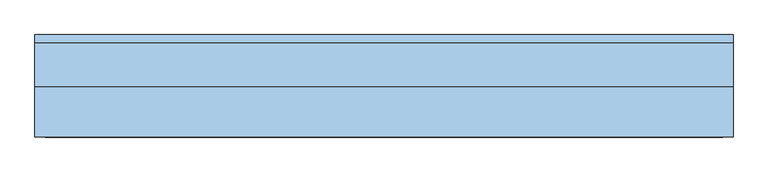
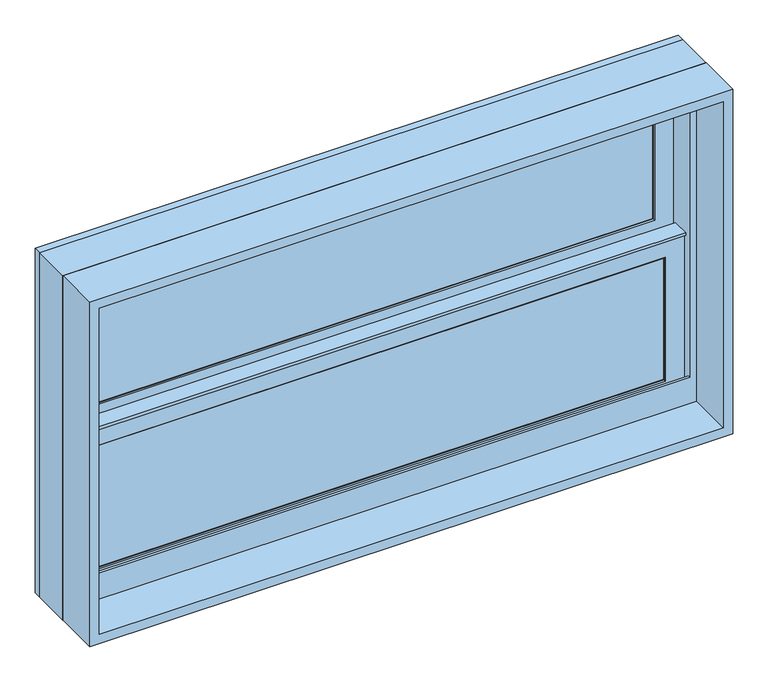
"""IFC4 building model written with IfcOpenShell, lengths in millimetres: window geometry, Window-Double_Hung-Marvin-Essential : ESDH3620."""

from ifc_helpers import new_model, si_unit, frame, origin, place, context, project, spatial, polyline, outline, extrude, faceted_brep, source, transform, mapped, element, save


def window_9b21e59f(model_context):
    return source(origin(), model_context, "Body", "SolidModel", [
        extrude(outline(polyline([(166.1583333, 20.6375), (166.1583333, 15.875), (147.1083333, 15.875), (147.1083333, 20.6375), (166.1583333, 20.6375)])), frame((0.0, 0.0, 1898.65), z_axis=(0.0, 0.0, 1.0), x_axis=(1.0, 0.0, 0.0)), (0.0, 0.0, 1.0), 222.25),
        extrude(outline(polyline([(-147.1083333, 20.6375), (-147.1083333, 15.875), (-166.1583333, 15.875), (-166.1583333, 20.6375), (-147.1083333, 20.6375)])), frame((0.0, 0.0, 1898.65), z_axis=(0.0, 0.0, 1.0), x_axis=(1.0, 0.0, 0.0)), (0.0, 0.0, 1.0), 222.25),
        extrude(outline(polyline([(469.9, 20.6375), (469.9, 15.875), (-469.9, 15.875), (-469.9, 20.6375), (469.9, 20.6375)])), frame((0.0, 0.0, 2000.25), z_axis=(0.0, 0.0, 1.0), x_axis=(1.0, 0.0, 0.0)), (0.0, 0.0, 1.0), 19.05),
        extrude(outline(polyline([(-166.1583333, 46.83125), (-166.1583333, 51.59375), (-147.1083333, 51.59375), (-147.1083333, 46.83125), (-166.1583333, 46.83125)])), frame((0.0, 0.0, 2159.0), z_axis=(0.0, 0.0, 1.0), x_axis=(1.0, 0.0, 0.0)), (0.0, 0.0, 1.0), 222.25),
        extrude(outline(polyline([(147.1083333, 46.83125), (147.1083333, 51.59375), (166.1583333, 51.59375), (166.1583333, 46.83125), (147.1083333, 46.83125)])), frame((0.0, 0.0, 2159.0), z_axis=(0.0, 0.0, 1.0), x_axis=(1.0, 0.0, 0.0)), (0.0, 0.0, 1.0), 222.25),
        extrude(outline(polyline([(-469.9, 46.83125), (-469.9, 51.59375), (469.9, 51.59375), (469.9, 46.83125), (-469.9, 46.83125)])), frame((0.0, 0.0, 2260.6), z_axis=(0.0, 0.0, 1.0), x_axis=(1.0, 0.0, 0.0)), (0.0, 0.0, 1.0), 19.05),
        extrude(outline(polyline([(166.1583333, 20.6375), (147.1083333, 20.6375), (147.1083333, 25.4), (166.1583333, 25.4), (166.1583333, 20.6375)])), frame((0.0, 0.0, 1898.65), z_axis=(0.0, 0.0, 1.0), x_axis=(1.0, 0.0, 0.0)), (0.0, 0.0, 1.0), 222.25),
        extrude(outline(polyline([(-147.1083333, 20.6375), (-166.1583333, 20.6375), (-166.1583333, 25.4), (-147.1083333, 25.4), (-147.1083333, 20.6375)])), frame((0.0, 0.0, 1898.65), z_axis=(0.0, 0.0, 1.0), x_axis=(1.0, 0.0, 0.0)), (0.0, 0.0, 1.0), 222.25),
        extrude(outline(polyline([(469.9, 20.6375), (-469.9, 20.6375), (-469.9, 25.4), (469.9, 25.4), (469.9, 20.6375)])), frame((0.0, 0.0, 2000.25), z_axis=(0.0, 0.0, 1.0), x_axis=(1.0, 0.0, 0.0)), (0.0, 0.0, 1.0), 19.05),
        extrude(outline(polyline([(-166.1583333, 56.35625), (-147.1083333, 56.35625), (-147.1083333, 51.59375), (-166.1583333, 51.59375), (-166.1583333, 56.35625)])), frame((0.0, 0.0, 2159.0), z_axis=(0.0, 0.0, 1.0), x_axis=(1.0, 0.0, 0.0)), (0.0, 0.0, 1.0), 222.25),
        extrude(outline(polyline([(147.1083333, 56.35625), (166.1583333, 56.35625), (166.1583333, 51.59375), (147.1083333, 51.59375), (147.1083333, 56.35625)])), frame((0.0, 0.0, 2159.0), z_axis=(0.0, 0.0, 1.0), x_axis=(1.0, 0.0, 0.0)), (0.0, 0.0, 1.0), 222.25),
        extrude(outline(polyline([(-469.9, 56.35625), (469.9, 56.35625), (469.9, 51.59375), (-469.9, 51.59375), (-469.9, 56.35625)])), frame((0.0, 0.0, 2260.6), z_axis=(0.0, 0.0, 1.0), x_axis=(1.0, 0.0, 0.0)), (0.0, 0.0, 1.0), 19.05),
        faceted_brep([(-496.8875, 5.6780605, 2150.9351748), (-496.8875, 5.6780605, 2146.3), (496.8875, 5.6780605, 2146.3), (496.8875, 5.6780605, 2150.9351748), (-496.8875, 34.8118605, 2150.9351748), (496.8875, 34.8118605, 2150.9351748), (496.8875, 34.8118605, 2146.3), (-496.8875, 34.8118605, 2146.3), (-496.8875, 30.1625, 2146.3), (-496.8875, 30.1625, 1871.6625), (-496.8875, 8.9241104, 1871.6625), (-496.8875, 8.9241104, 2146.3), (496.8875, 8.9241104, 2146.3), (496.8875, 30.1625, 2146.3), (496.8875, 8.9241104, 1871.6625), (496.8875, 30.1625, 1871.6625), (-481.0034752, 11.90625, 2132.0034752), (-481.0034752, 30.1625, 2132.0034752), (481.0034752, 30.1625, 2132.0034752), (481.0034752, 11.90625, 2132.0034752), (-464.34375, 10.4662439, 2115.34375), (-464.34375, 11.90625, 2115.34375), (464.34375, 11.90625, 2115.34375), (464.34375, 10.4662439, 2115.34375), (465.8858834, 8.9241104, 2116.8858834), (-465.8858834, 8.9241104, 2116.8858834), (481.0034752, 30.1625, 1887.5465248), (481.0034752, 11.90625, 1887.5465248), (464.34375, 11.90625, 1904.20625), (464.34375, 10.4662439, 1904.20625), (465.8858834, 8.9241104, 1902.6641166), (-481.0034752, 30.1625, 1887.5465248), (-481.0034752, 11.90625, 1887.5465248), (-464.34375, 11.90625, 1904.20625), (-464.34375, 10.4662439, 1904.20625), (-465.8858834, 8.9241104, 1902.6641166)], [[[0, 1, 2, 3]], [[4, 5, 6, 7]], [[1, 0, 4, 7, 8, 9, 10, 11]], [[2, 1, 11, 12]], [[7, 6, 13, 8]], [[3, 2, 12, 14, 15, 13, 6, 5]], [[0, 3, 5, 4]], [[16, 17, 18, 19]], [[20, 21, 22, 23]], [[20, 23, 24, 25]], [[19, 18, 26, 27]], [[23, 22, 28, 29]], [[24, 23, 29, 30]], [[27, 26, 31, 32]], [[29, 28, 33, 34]], [[30, 29, 34, 35]], [[15, 14, 10, 9]], [[15, 9, 8, 13], [18, 17, 31, 26]], [[17, 16, 32, 31]], [[16, 19, 27, 32], [22, 21, 33, 28]], [[21, 20, 34, 33]], [[20, 25, 35, 34]], [[10, 14, 12, 11], [25, 24, 30, 35]]]),
        extrude(outline(polyline([(38.5955581, 2132.0125), (33.5778968, 2132.0125), (33.5778968, 2133.6), (39.9405976, 2133.6), (39.9405976, 2132.0125), (61.515625, 2132.0125), (47.6307501, 2128.6975159), (38.5955581, 2128.6975159), (38.5955581, 2132.0125)])), frame((-496.8875, 0.0, 0.0), z_axis=(1.0, 0.0, 0.0), x_axis=(0.0, 1.0, 0.0)), (0.0, 0.0, 1.0), 993.775),
        faceted_brep([(527.05, 0.0, 1841.5), (527.05, 0.0, 2438.4), (-527.05, 0.0, 2438.4), (-527.05, 0.0, 1841.5), (500.85625, 0.0, 1902.61875), (-500.85625, 0.0, 1902.61875), (-500.85625, 0.0, 2412.20625), (500.85625, 0.0, 2412.20625), (500.85625, 3.96875, 1841.5), (-500.85625, 3.96875, 1841.5), (-500.85625, 3.96875, 1902.61875), (500.85625, 3.96875, 1902.61875), (-527.05, 65.6828125, 1841.5), (-500.85625, 65.6828125, 1841.5), (500.85625, 65.6828125, 1841.5), (527.05, 65.6828125, 1841.5), (-527.05, 65.6828125, 2438.4), (527.05, 65.6828125, 2438.4), (500.85625, 65.6828125, 2412.20625), (-500.85625, 65.6828125, 2412.20625)], [[[0, 1, 2, 3], [4, 5, 6, 7]], [[8, 9, 10, 11]], [[5, 4, 11, 10]], [[0, 3, 12, 13, 9, 8, 14, 15]], [[13, 12, 16, 17, 15, 14, 18, 19]], [[13, 19, 6, 5, 10, 9]], [[7, 6, 19, 18]], [[18, 14, 8, 11, 4, 7]], [[1, 0, 15, 17]], [[2, 1, 17, 16]], [[3, 2, 16, 12]]]),
        faceted_brep([(500.85625, 30.1625, 2139.95), (499.26875, 30.1625, 2139.95), (499.26875, 30.1625, 1865.8544613), (500.85625, 30.1625, 1865.8544613), (-499.26875, 30.1625, 2139.95), (-500.85625, 30.1625, 2139.95), (-500.85625, 30.1625, 1865.8544613), (-499.26875, 30.1625, 1865.8544613), (499.26875, 63.5, 2139.95), (500.85625, 63.5, 2139.95), (500.85625, 63.5, 1859.3743077), (499.26875, 63.5, 1859.3743077), (-500.85625, 63.5, 2139.95), (-499.26875, 63.5, 2139.95), (-499.26875, 63.5, 1859.3743077), (-500.85625, 63.5, 1859.3743077), (512.1108932, 3.96875, 1870.9460105), (512.1108932, 3.96875, 1841.5), (512.1108932, 65.6828125, 1841.5), (512.1108932, 65.6828125, 1858.950012), (-512.1108932, 3.96875, 1841.5), (-512.1108932, 3.96875, 1870.9460105), (-512.1108932, 65.6828125, 1858.950012), (-512.1108932, 65.6828125, 1841.5), (512.1108932, 78.58125, 1856.4428097), (-512.1108932, 78.58125, 1856.4428097), (-510.0971252, 68.2348864, 1858.4539391), (-492.13135, 68.2348864, 1858.4539391), (-492.13135, 65.6828125, 1858.950012), (492.13135, 65.6828125, 1858.950012), (492.13135, 68.2348864, 1858.4539391), (510.0971252, 68.2348864, 1858.4539391), (-527.05, 65.6828125, 1841.5), (-527.05, 78.5948249, 1841.5), (527.05, 78.5948249, 1841.5), (527.05, 65.6828125, 1841.5), (-527.05, 78.58125, 2438.4), (527.05, 78.58125, 2438.4), (512.1108932, 78.58125, 2423.4608932), (-512.1108932, 78.58125, 2423.4608932), (-527.05, 65.6828125, 2438.4), (-510.0971252, 68.2348864, 2421.4471252), (510.0971252, 68.2348864, 2421.4471252), (492.13135, 68.2348864, 2403.48135), (-492.13135, 68.2348864, 2403.48135), (-492.13135, 65.6828125, 2403.48135), (492.13135, 65.6828125, 2403.48135), (527.05, 65.6828125, 2438.4)], [[[0, 1, 2, 3]], [[4, 5, 6, 7]], [[8, 9, 10, 11]], [[12, 13, 14, 15]], [[1, 8, 11, 2]], [[9, 0, 3, 10]], [[1, 0, 9, 8]], [[5, 4, 13, 12]], [[5, 12, 15, 6]], [[13, 4, 7, 14]], [[16, 17, 18, 19]], [[20, 21, 22, 23]], [[24, 25, 26, 27, 28, 22, 21, 16, 19, 29, 30, 31], [3, 2, 11, 10], [7, 6, 15, 14]], [[17, 16, 21, 20]], [[17, 20, 23, 32, 33, 34, 35, 18]], [[34, 33, 36, 37], [25, 24, 38, 39]], [[33, 32, 40, 36]], [[39, 41, 26, 25]], [[41, 42, 31, 30, 43, 44, 27, 26]], [[44, 45, 28, 27]], [[40, 32, 23, 22, 28, 45, 46, 29, 19, 18, 35, 47]], [[36, 40, 47, 37]], [[39, 38, 42, 41]], [[44, 43, 46, 45]], [[34, 37, 47, 35]], [[42, 38, 24, 31]], [[46, 43, 30, 29]]]),
        extrude(outline(polyline([(477.04375, 11.90625), (-477.04375, 11.90625), (-477.04375, 15.08125), (477.04375, 15.08125), (477.04375, 11.90625)])), frame((0.0, 0.0, 1891.50625), z_axis=(0.0, 0.0, 1.0), x_axis=(1.0, 0.0, 0.0)), (0.0, 0.0, 1.0), 236.5375),
        extrude(outline(polyline([(477.04375, 42.8625), (-477.04375, 42.8625), (-477.04375, 46.0375), (477.04375, 46.0375), (477.04375, 42.8625)])), frame((0.0, 0.0, 2151.85625), z_axis=(0.0, 0.0, 1.0), x_axis=(1.0, 0.0, 0.0)), (0.0, 0.0, 1.0), 236.5375),
        faceted_brep([(-464.34375, 31.194477, 2115.34375), (-465.8858834, 32.7366104, 2116.8858834), (465.8858834, 32.7366104, 2116.8858834), (464.34375, 31.194477, 2115.34375), (-464.34375, 30.1625, 2115.34375), (464.34375, 30.1625, 2115.34375), (-496.8875, 32.7366104, 2147.8875), (-496.8875, 30.1625, 2147.8875), (496.8875, 30.1625, 2147.8875), (496.8875, 32.7366104, 2147.8875), (465.8858834, 32.7366104, 1902.6641166), (464.34375, 31.194477, 1904.20625), (464.34375, 30.1625, 1904.20625), (496.8875, 30.1625, 1871.6625), (496.8875, 32.7366104, 1871.6625), (-465.8858834, 32.7366104, 1902.6641166), (-464.34375, 31.194477, 1904.20625), (-464.34375, 30.1625, 1904.20625), (-496.8875, 30.1625, 1871.6625), (-496.8875, 32.7366104, 1871.6625)], [[[0, 1, 2, 3]], [[4, 0, 3, 5]], [[6, 7, 8, 9]], [[3, 2, 10, 11]], [[5, 3, 11, 12]], [[9, 8, 13, 14]], [[11, 10, 15, 16]], [[12, 11, 16, 17]], [[14, 13, 18, 19]], [[9, 14, 19, 6], [1, 15, 10, 2]], [[16, 15, 1, 0]], [[17, 16, 0, 4]], [[7, 18, 13, 8], [5, 12, 17, 4]], [[19, 18, 7, 6]]]),
        faceted_brep([(-481.0034752, 42.8625, 2392.3534752), (-481.0034752, 61.11875, 2392.3534752), (481.0034752, 61.11875, 2392.3534752), (481.0034752, 42.8625, 2392.3534752), (-464.34375, 41.4224939, 2375.69375), (-464.34375, 42.8625, 2375.69375), (464.34375, 42.8625, 2375.69375), (464.34375, 41.4224939, 2375.69375), (-465.8858834, 39.8803604, 2377.2358834), (465.8858834, 39.8803604, 2377.2358834), (-496.8875, 61.11875, 2408.2375), (-496.8875, 39.8803604, 2408.2375), (496.8875, 39.8803604, 2408.2375), (496.8875, 61.11875, 2408.2375), (481.0034752, 61.11875, 2147.8965248), (481.0034752, 42.8625, 2147.8965248), (464.34375, 42.8625, 2164.55625), (464.34375, 41.4224939, 2164.55625), (465.8858834, 39.8803604, 2163.0141166), (496.8875, 39.8803604, 2132.0125), (496.8875, 61.11875, 2132.0125), (-481.0034752, 61.11875, 2147.8965248), (-481.0034752, 42.8625, 2147.8965248), (-464.34375, 42.8625, 2164.55625), (-464.34375, 41.4224939, 2164.55625), (-465.8858834, 39.8803604, 2163.0141166), (-496.8875, 39.8803604, 2132.0125), (-496.8875, 61.11875, 2132.0125)], [[[0, 1, 2, 3]], [[4, 5, 6, 7]], [[8, 4, 7, 9]], [[10, 11, 12, 13]], [[3, 2, 14, 15]], [[7, 6, 16, 17]], [[9, 7, 17, 18]], [[13, 12, 19, 20]], [[15, 14, 21, 22]], [[17, 16, 23, 24]], [[18, 17, 24, 25]], [[20, 19, 26, 27]], [[13, 20, 27, 10], [1, 21, 14, 2]], [[22, 21, 1, 0]], [[3, 15, 22, 0], [5, 23, 16, 6]], [[24, 23, 5, 4]], [[25, 24, 4, 8]], [[11, 26, 19, 12], [9, 18, 25, 8]], [[27, 26, 11, 10]]]),
        faceted_brep([(-496.8875, 61.11875, 2132.0125), (-496.8875, 63.6928604, 2132.0125), (496.8875, 63.6928604, 2132.0125), (496.8875, 61.11875, 2132.0125), (-464.34375, 62.150727, 2164.55625), (-464.34375, 61.11875, 2164.55625), (464.34375, 61.11875, 2164.55625), (464.34375, 62.150727, 2164.55625), (-465.8858834, 63.6928604, 2163.0141166), (465.8858834, 63.6928604, 2163.0141166), (496.8875, 63.6928604, 2408.2375), (496.8875, 61.11875, 2408.2375), (464.34375, 61.11875, 2375.69375), (464.34375, 62.150727, 2375.69375), (465.8858834, 63.6928604, 2377.2358834), (-496.8875, 63.6928604, 2408.2375), (-496.8875, 61.11875, 2408.2375), (-464.34375, 61.11875, 2375.69375), (-464.34375, 62.150727, 2375.69375), (-465.8858834, 63.6928604, 2377.2358834)], [[[0, 1, 2, 3]], [[4, 5, 6, 7]], [[8, 4, 7, 9]], [[3, 2, 10, 11]], [[7, 6, 12, 13]], [[9, 7, 13, 14]], [[11, 10, 15, 16]], [[13, 12, 17, 18]], [[14, 13, 18, 19]], [[16, 15, 1, 0]], [[3, 11, 16, 0], [5, 17, 12, 6]], [[18, 17, 5, 4]], [[19, 18, 4, 8]], [[1, 15, 10, 2], [9, 14, 19, 8]]]),
        extrude(outline(polyline([(477.04375, 26.19375), (-477.04375, 26.19375), (-477.04375, 30.1625), (477.04375, 30.1625), (477.04375, 26.19375)])), frame((0.0, 0.0, 1891.50625), z_axis=(0.0, 0.0, 1.0), x_axis=(1.0, 0.0, 0.0)), (0.0, 0.0, 1.0), 236.5375),
        extrude(outline(polyline([(477.04375, 57.15), (-477.04375, 57.15), (-477.04375, 61.11875), (477.04375, 61.11875), (477.04375, 57.15)])), frame((0.0, 0.0, 2151.85625), z_axis=(0.0, 0.0, 1.0), x_axis=(1.0, 0.0, 0.0)), (0.0, 0.0, 1.0), 236.5375),
        extrude(outline(polyline([(2438.4, 527.05), (2438.4, -527.05), (1841.5, -527.05), (1841.5, 527.05), (2438.4, 527.05)]), holes=[polyline([(2422.525, 511.175), (1857.375, 511.175), (1857.375, -511.175), (2422.525, -511.175), (2422.525, 511.175)])]), frame((0.0, -76.2, 0.0), z_axis=(0.0, 1.0, 0.0), x_axis=(0.0, 0.0, 1.0)), (0.0, 0.0, 1.0), 75.40625),
    ])


if __name__ == "__main__":
    model = new_model("IFC4")
    model_context = context("Model", 3, world=origin())
    ifc_project = project(units=[si_unit("LENGTHUNIT", "METRE", prefix="MILLI")], contexts=[model_context])
    site = spatial("IfcSite", under=ifc_project)
    building = spatial("IfcBuilding", under=site)
    placement = place(None, origin())
    window_shape = window_9b21e59f(model_context)
    element("IfcWindow", 1, ObjectType="Window-Double_Hung-Marvin-Essential : ESDH3620", at=placement, inside=building, context=model_context, shape_type="MappedRepresentation", body=[
        mapped(window_shape, transform((0.0, 0.0, 0.0), x_axis=(1.0, 0.0, 0.0), y_axis=(0.0, 1.0, 0.0), z_axis=(0.0, 0.0, 1.0))),
    ])
    save(model, "model.ifc")

# Revit data of these elements
# Type "Window-Double_Hung-Marvin-Essential : ESDH3620"
#   Type Mark = "24"
#   Window Type = "Essential Double Hung"
#   Product data url = "https://bimobject.com/marvin-windows-and-doors/product/marvin-dhwau"
#   Product Guid = "c4a96547-874c-4385-91dc-a058adc19d98"
#   Frame = "All Ultrex"
#   Egress Window = "No"
#   URL = "www.marvin.com"
#   Model = "ESDH3620"
#   Manufacturer = "Marvin Windows and Doors"
#   Label Egress = ""
#   Glass Type = "IG Low E II with Argon"
#   Design Pressure = "DP50"
#   Description = "4224 DBHG"
#   Analytic Construction = "<None>"
#   Prairie Corner Width = 0' - 4"
#   Prairie Corner Height = 0' - 4"
#   Egress Width = 3' - 2 9/16"
#   Egress Height = 0' - 7 27/128"
#   Rough Width = 3' - 6"
#   Rough Height = 2' - 0"
#   Nominal Width = 3' - 6"
#   Nominal Height = 2' - 0"
#   Inset to Installation Flange [instance default] = 0' - 1"
#   Height = 1' - 11 1/2"
#   Egress Area = 1.93105 SF
#   Default Head Height = 8' - 0"
#   Width = 3' - 5 1/2"
#   Daylight Area = 4.22119 SF
#   DLO Width = 3' - 0 9/16"
#   DLO Height = 0' - 8 5/16"
#   Muntins Top Sash = yes
#   Lites Wide Top Sash = 3
#   Lites Wide Bottom Sash = 3
#   Lites High Top Sash = 2
#   Lites High Bottom Sash = 2
#   Lite Cut Prairie 9 = no
#   Lite Cut HV Grid = yes
#   Muntins Bottom Sash = yes
#   Label Visibility = no
#   Jamb Extension Visibility = yes
#   Edition number = 1
#   Interior Material = Ultrex-Marvin-Stonewhite
#   Glazing Material = Glass-Marvin-IG Low E II with Argon
#   Cladding Material = Ultrex-Marvin-Pebblegray
#   Wall Closure = (empty or 0)
#   Assembly Code = ""
# Element 1 (IfcWindow, "Window-Double_Hung-Marvin-Essential : ESDH3620")
#   Materials on its faces: "Ultrex-Marvin-Pebblegray", "Ultrex-Marvin-Stonewhite", "Glass-Marvin-IG Low E II with Argon"
# Materials
#   "Ultrex-Marvin-Stonewhite": class "Paint", colour RGB 250 251 245, transparency 0
#   "Glass-Marvin-IG Low E II with Argon": class "Glass", colour RGB 0 128 192, transparency 0.85
#   "Ultrex-Marvin-Pebblegray": class "Paint", colour RGB 189 185 173, transparency 0
